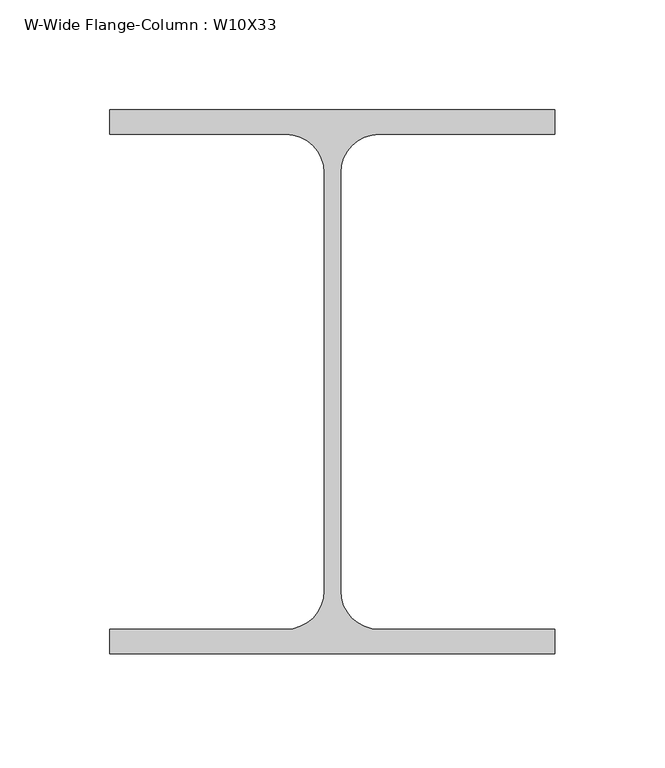
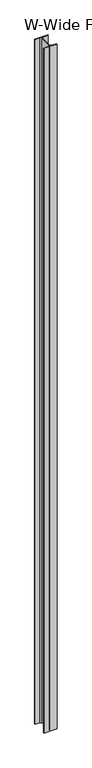
"""IFC4 building model written with IfcOpenShell, lengths in millimetres: column geometry, W-Wide Flange-Column : W10X33."""

import ifcopenshell
import ifcopenshell.guid

model = None  # the IFC model being written
_history = None  # IfcOwnerHistory: only IFC2X3 demands one
_inside = {}  # id of a spatial element -> (the spatial element, [elements in it])
_under = {}  # id of a project, library or spatial element -> (it, [spatial elements below it])
_declared = {}  # id of a project -> (the project, [libraries it declares])
_typed = {}  # id of a type object -> (the type object, [elements of that type])
_made_of = {}  # id of a material, layer set ... -> (it, [elements and type objects made of it])


def new_model(schema):
    """Start an empty IFC model of exactly this schema.

    Asked for "IFC4X3", IfcOpenShell would pick the latest addendum, in which some entities
    have other attributes; the version numbers below select the first issue.
    IFC2X3 requires an IfcOwnerHistory on every rooted entity: one is made here for all.
    """
    global model, _history
    if schema == "IFC4X3":
        model = ifcopenshell.file(schema_version=(4, 3, 0, 0))
    else:
        model = ifcopenshell.file(schema=schema)
    _inside.clear()
    _under.clear()
    _declared.clear()
    _typed.clear()
    _made_of.clear()
    _history = None
    if model.schema == "IFC2X3":
        org = make("IfcOrganization", Name="unknown")
        user = make(
            "IfcPersonAndOrganization",
            ThePerson=make("IfcPerson", FamilyName="unknown"),
            TheOrganization=org,
        )
        app = make(
            "IfcApplication",
            ApplicationDeveloper=org,
            Version="unknown",
            ApplicationFullName="unknown",
            ApplicationIdentifier="unknown",
        )
        _history = make(
            "IfcOwnerHistory",
            OwningUser=user,
            OwningApplication=app,
            ChangeAction="ADDED",
            CreationDate=0,
        )
    return model


def make(cls, **values):
    """One entity of the class cls with the attributes given. An attribute that is None is left unset."""
    return model.create_entity(
        cls, **{name: value for name, value in values.items() if value is not None}
    )


def rooted(cls, **values):
    """An entity with a GlobalId (a new one), such as an element, a storey or a relation."""
    return make(cls, GlobalId=ifcopenshell.guid.new(), OwnerHistory=_history, **values)


def si_unit(unit_type, name, prefix=None):
    """IfcSIUnit, for example si_unit("LENGTHUNIT", "METRE", prefix="MILLI")."""
    return make("IfcSIUnit", UnitType=unit_type, Prefix=prefix, Name=name)


def assignment(units):
    """IfcUnitAssignment: the units of a project."""
    return None if units is None else make("IfcUnitAssignment", Units=units)


def point(xyz):
    """IfcCartesianPoint."""
    return None if xyz is None else make("IfcCartesianPoint", Coordinates=xyz)


def direction(xyz):
    """IfcDirection."""
    return None if xyz is None else make("IfcDirection", DirectionRatios=xyz)


def frame(location, z_axis=None, x_axis=None):
    """IfcAxis2Placement3D, a coordinate frame: its origin and axes. An axis left out is left unset."""
    return make(
        "IfcAxis2Placement3D",
        Location=point(location),
        Axis=direction(z_axis),
        RefDirection=direction(x_axis),
    )


def frame_2d(location, x_axis=None):
    """IfcAxis2Placement2D, a coordinate frame in the plane: its origin and x axis."""
    return make(
        "IfcAxis2Placement2D", Location=point(location), RefDirection=direction(x_axis)
    )


def origin():
    """The frame at (0, 0, 0) with its axes left unset."""
    return frame((0.0, 0.0, 0.0))


def place(relative_to, where):
    """IfcLocalPlacement: puts the frame where relative to a parent placement (None: the world)."""
    return make(
        "IfcLocalPlacement", PlacementRelTo=relative_to, RelativePlacement=where
    )


def context(
    kind, dimensions, precision=None, world=None, true_north=None, identifier=None
):
    """IfcGeometricRepresentationContext, for example the 3D "Model" context."""
    return make(
        "IfcGeometricRepresentationContext",
        ContextIdentifier=identifier,
        ContextType=kind,
        CoordinateSpaceDimension=dimensions,
        Precision=precision,
        WorldCoordinateSystem=world,
        TrueNorth=true_north,
    )


def project(units=None, contexts=None):
    """IfcProject with its units and contexts."""
    return rooted(
        "IfcProject",
        Name="project",
        RepresentationContexts=contexts,
        UnitsInContext=assignment(units),
    )


def spatial(cls, under=None, at=None, **own):
    """A site, building, storey or space (cls), placed at a placement, below another one or the project."""
    s = rooted(cls, ObjectPlacement=at, **own)
    if under is not None:
        _under.setdefault(under.id(), (under, []))[1].append(s)
    return s


def polyline(points):
    """IfcPolyline through the points."""
    return make("IfcPolyline", Points=[point(p) for p in points])


def circle_curve(where, radius):
    """IfcCircle in the frame where."""
    return make("IfcCircle", Position=where, Radius=radius)


def trimmed(basis, trim1, trim2, sense, master):
    """IfcTrimmedCurve: the piece of a basis curve between two trims."""
    return make(
        "IfcTrimmedCurve",
        BasisCurve=basis,
        Trim1=trim1,
        Trim2=trim2,
        SenseAgreement=sense,
        MasterRepresentation=master,
    )


def segment(curve, same_sense, transition):
    """IfcCompositeCurveSegment."""
    return make(
        "IfcCompositeCurveSegment",
        Transition=transition,
        SameSense=same_sense,
        ParentCurve=curve,
    )


def composite_curve(segments, self_intersect=None):
    """IfcCompositeCurve: segments joined end to end."""
    return make("IfcCompositeCurve", Segments=segments, SelfIntersect=self_intersect)


def outline(outer, holes=None, kind="AREA"):
    """IfcArbitraryClosedProfileDef: a profile drawn as a closed curve; with holes, ...WithVoids."""
    if holes is None:
        return make("IfcArbitraryClosedProfileDef", ProfileType=kind, OuterCurve=outer)
    return make(
        "IfcArbitraryProfileDefWithVoids",
        ProfileType=kind,
        OuterCurve=outer,
        InnerCurves=holes,
    )


def extrude(swept, where, along, depth):
    """IfcExtrudedAreaSolid: the profile swept, set in the frame where, extruded along a direction by depth."""
    return make(
        "IfcExtrudedAreaSolid",
        SweptArea=swept,
        Position=where,
        ExtrudedDirection=direction(along),
        Depth=depth,
    )


def shape(context_of_items, identifier, shape_type, items):
    """IfcShapeRepresentation: the items that make up one representation, for example the "Body"."""
    return make(
        "IfcShapeRepresentation",
        ContextOfItems=context_of_items,
        RepresentationIdentifier=identifier,
        RepresentationType=shape_type,
        Items=items,
    )


def source(mapping_origin, context_of_items, identifier, shape_type, items):
    """IfcRepresentationMap: a shape defined once, which mapped items show again and again."""
    return make(
        "IfcRepresentationMap",
        MappingOrigin=mapping_origin,
        MappedRepresentation=shape(context_of_items, identifier, shape_type, items),
    )


def transform(
    local_origin,
    x_axis=None,
    y_axis=None,
    z_axis=None,
    scale=None,
    scale2=None,
    scale3=None,
    uniform=True,
):
    """IfcCartesianTransformationOperator3D, or its non-uniform kind. x_axis, y_axis, z_axis: its Axis1, 2, 3."""
    if uniform:
        return make(
            "IfcCartesianTransformationOperator3D",
            Axis1=direction(x_axis),
            Axis2=direction(y_axis),
            LocalOrigin=point(local_origin),
            Scale=scale,
            Axis3=direction(z_axis),
        )
    return make(
        "IfcCartesianTransformationOperator3DnonUniform",
        Axis1=direction(x_axis),
        Axis2=direction(y_axis),
        LocalOrigin=point(local_origin),
        Scale=scale,
        Axis3=direction(z_axis),
        Scale2=scale2,
        Scale3=scale3,
    )


def mapped(mapping_source, mapping_target):
    """IfcMappedItem: shows the shape of a source again, moved by a transform."""
    return make(
        "IfcMappedItem", MappingSource=mapping_source, MappingTarget=mapping_target
    )


def made_of(thing, what):
    """Note that an element or type object is made of a material, layer set ...; save() writes the relation."""
    if what is not None:
        _made_of.setdefault(what.id(), (what, []))[1].append(thing)
    return thing


def element(
    cls,
    number,
    at=None,
    inside=None,
    cuts=None,
    type_object=None,
    material=None,
    context=None,
    identifier="Body",
    shape_type=None,
    held_by="IfcProductDefinitionShape",
    body=None,
    shapes=None,
    **own,
):
    """One element of the class cls, such as IfcWall. Its Tag is "e" and its number.

    at: its placement. inside: the storey or other place that contains it. cuts: it is an
    opening in that element (IfcRelVoidsElement). A single representation is given by context,
    identifier, shape_type and body (its items); several are given by shapes. held_by: the class
    of the entity that holds the representations. save() writes the other relations.
    """
    e = rooted(cls, Tag="e%d" % number, ObjectPlacement=at, **own)
    if body is not None:
        shapes = [shape(context, identifier, shape_type, body)]
    if shapes is not None:
        e.Representation = make(held_by, Representations=shapes)
    if inside is not None:
        _inside.setdefault(inside.id(), (inside, []))[1].append(e)
    if cuts is not None:
        rooted(
            "IfcRelVoidsElement", RelatingBuildingElement=cuts, RelatedOpeningElement=e
        )
    if type_object is not None:
        _typed.setdefault(type_object.id(), (type_object, []))[1].append(e)
    return made_of(e, material)


def aggregate(whole, parts):
    """IfcRelAggregates: a whole, such as a stair, and the parts it consists of."""
    return rooted("IfcRelAggregates", RelatingObject=whole, RelatedObjects=parts)


def save(model, path):
    """Write the relations noted so far, then the file.

    IfcRelAggregates (storeys below a building ...), IfcRelContainedInSpatialStructure (elements
    in a storey), IfcRelDefinesByType, IfcRelAssociatesMaterial and IfcRelDeclares: one each for
    every whole, place, type object, material and project.
    """
    for whole, parts in _under.values():
        aggregate(whole, parts)
    for where, things in _inside.values():
        rooted(
            "IfcRelContainedInSpatialStructure",
            RelatedElements=things,
            RelatingStructure=where,
        )
    for kind, things in _typed.values():
        rooted("IfcRelDefinesByType", RelatedObjects=things, RelatingType=kind)
    for what, things in _made_of.values():
        rooted("IfcRelAssociatesMaterial", RelatedObjects=things, RelatingMaterial=what)
    for by, libraries in _declared.values():
        rooted("IfcRelDeclares", RelatingContext=by, RelatedDefinitions=libraries)
    model.write(path)


def w_wide_flange_column_w10x33_a2e74f78(model_context):
    return source(origin(), model_context, "Body", "SweptSolid", [
        extrude(outline(composite_curve([segment(polyline([(101.092, 123.571), (101.092, 112.522), (21.209, 112.522)]), True, "CONTINUOUS"), segment(trimmed(circle_curve(frame_2d((21.209, 94.996)), 17.526), [point((21.209, 112.522))], [point((3.683, 94.996))], True, "CARTESIAN"), True, "CONTINUOUS"), segment(polyline([(3.683, 94.996), (3.683, -94.996)]), True, "CONTINUOUS"), segment(trimmed(circle_curve(frame_2d((21.209, -94.996)), 17.526), [point((3.683, -94.996))], [point((21.209, -112.522))], True, "CARTESIAN"), True, "CONTINUOUS"), segment(polyline([(21.209, -112.522), (101.092, -112.522), (101.092, -123.571), (-101.092, -123.571), (-101.092, -112.522), (-21.209, -112.522)]), True, "CONTINUOUS"), segment(trimmed(circle_curve(frame_2d((-21.209, -94.996)), 17.526), [point((-21.209, -112.522))], [point((-3.683, -94.996))], True, "CARTESIAN"), True, "CONTINUOUS"), segment(polyline([(-3.683, -94.996), (-3.683, 94.996)]), True, "CONTINUOUS"), segment(trimmed(circle_curve(frame_2d((-21.209, 94.996)), 17.526), [point((-3.683, 94.996))], [point((-21.209, 112.522))], True, "CARTESIAN"), True, "CONTINUOUS"), segment(polyline([(-21.209, 112.522), (-101.092, 112.522), (-101.092, 123.571), (101.092, 123.571)]), True, "CONTINUOUS")], self_intersect=False)), frame((0.0, 0.0, 16408.4), z_axis=(0.0, 0.0, 1.0), x_axis=(1.0, 0.0, 0.0)), (0.0, 0.0, 1.0), 11176.0),
    ])


if __name__ == "__main__":
    model = new_model("IFC4")
    model_context = context("Model", 3, world=origin())
    ifc_project = project(units=[si_unit("LENGTHUNIT", "METRE", prefix="MILLI")], contexts=[model_context])
    site = spatial("IfcSite", under=ifc_project)
    building = spatial("IfcBuilding", under=site)
    placement = place(None, origin())
    w_wide_flange_column_w10x33_shape = w_wide_flange_column_w10x33_a2e74f78(model_context)
    element("IfcColumn", 1, ObjectType="W-Wide Flange-Column : W10X33", at=placement, inside=building, context=model_context, shape_type="MappedRepresentation", body=[
        mapped(w_wide_flange_column_w10x33_shape, transform((0.0, 0.0, 0.0), x_axis=(1.0, 0.0, 0.0), y_axis=(0.0, 1.0, 0.0), z_axis=(0.0, 0.0, 1.0))),
    ])
    save(model, "model.ifc")

# Revit data of these elements
# Type "W-Wide Flange-Column : W10X33"
#   Assembly Code = "B10"
#   W = 33
#   bf = 0' - 7.96"
#   d = 0' - 9.73"
#   k = 0' - 1 1/8"
#   kr = 0' - 0.69"
#   tf = 0' - 0.435"
#   tw = 0' - 0.29"
#   A = 0.0674306 SF
#   Structural Material [instance default] = Steel ASTM A992
# Element 1 (IfcColumn, "W-Wide Flange-Column : W10X33")
#   Materials on its faces: "Steel ASTM A992"
# Materials
#   "Steel ASTM A992": class "Metal", colour RGB 199 199 199, transparency 0, Description = "Structural steel 50ksi", Cost = 0
